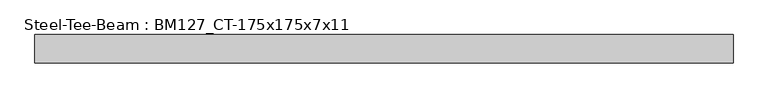
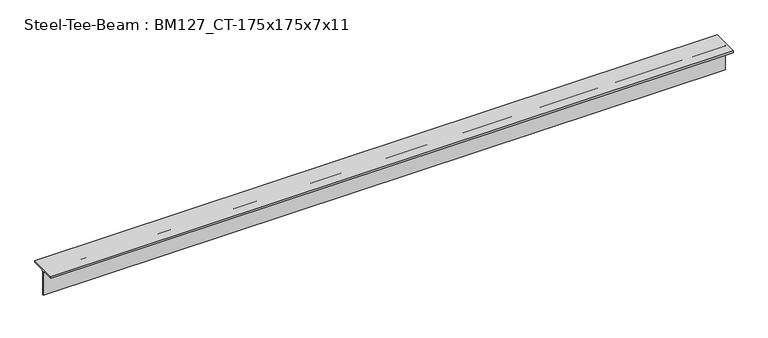
"""IFC4 building model written with IfcOpenShell, lengths in millimetres: beam geometry, Steel-Tee-Beam : BM127_CT-175x175x7x11."""

from ifc_helpers import new_model, si_unit, point, frame, frame_2d, origin, place, context, project, spatial, polyline, circle_curve, trimmed, segment, composite_curve, outline, extrude, source, transform, mapped, element, save


def steel_tee_beam_bm127_ct_175x175x7x11_73a373e1(model_context):
    return source(origin(), model_context, "Body", "SweptSolid", [
        extrude(outline(composite_curve([segment(polyline([(87.5, 87.5), (87.5, 76.5), (17.5, 76.5)]), True, "CONTINUOUS"), segment(trimmed(circle_curve(frame_2d((17.5, 62.5)), 14.0), [point((17.5, 76.5))], [point((3.5, 62.5))], True, "CARTESIAN"), True, "CONTINUOUS"), segment(polyline([(3.5, 62.5), (3.5, -87.5), (-3.5, -87.5), (-3.5, 62.5)]), True, "CONTINUOUS"), segment(trimmed(circle_curve(frame_2d((-17.5, 62.5)), 14.0), [point((-3.5, 62.5))], [point((-17.5, 76.5))], True, "CARTESIAN"), True, "CONTINUOUS"), segment(polyline([(-17.5, 76.5), (-87.5, 76.5), (-87.5, 87.5), (87.5, 87.5)]), True, "CONTINUOUS")], self_intersect=False)), frame((-2105.3835132, 0.0, 0.0), z_axis=(1.0, 0.0, 0.0), x_axis=(0.0, 1.0, 0.0)), (0.0, 0.0, 1.0), 4289.6201558),
    ])


if __name__ == "__main__":
    model = new_model("IFC4")
    model_context = context("Model", 3, world=origin())
    ifc_project = project(units=[si_unit("LENGTHUNIT", "METRE", prefix="MILLI")], contexts=[model_context])
    site = spatial("IfcSite", under=ifc_project)
    building = spatial("IfcBuilding", under=site)
    placement = place(None, origin())
    steel_tee_beam_bm127_ct_175x175x7x11_shape = steel_tee_beam_bm127_ct_175x175x7x11_73a373e1(model_context)
    element("IfcBeam", 1, ObjectType="Steel-Tee-Beam : BM127_CT-175x175x7x11", at=placement, inside=building, context=model_context, shape_type="MappedRepresentation", body=[
        mapped(steel_tee_beam_bm127_ct_175x175x7x11_shape, transform((0.0, 0.0, 0.0), x_axis=(1.0, 0.0, 0.0), y_axis=(0.0, 1.0, 0.0), z_axis=(0.0, 0.0, 1.0))),
    ])
    save(model, "model.ifc")

# Revit data of these elements
# Type "Steel-Tee-Beam : BM127_CT-175x175x7x11"
#   Surface Area = 0.00 m²/m
#   Section Area = 31.57 cm²
#   Mass per Unit Length = 24.80 kg/m
#   Length [instance default] = 1524 mm
#   bf = 175 mm
#   d = 175 mm
#   k = 25 mm
#   kr = 14 mm
#   tf = 11 mm
#   tw = 7 mm
#   hec_material4 [instance default] = none
#   hec_material3 [instance default] = none
#   hec_material2 [instance default] = none
#   hec_material1 [instance default] = none
#   Structural Material [instance default] = Steel, 45-345
#   Assembly Code = ""
# Element 1 (IfcBeam, "Steel-Tee-Beam : BM127_CT-175x175x7x11")
#   hec_material3 = F01AC000-00002_Building/Shelter Fire Proofing Work_Intumescent Coating Type_1 hr. rating (UL 1709))
#   hec_material2 = S01AA010-00002_Main Steel Structure Fabrication Work_Shelter/Building_Steel Painting/Coating_for Fireproofed Steel Surface, Surface Preparation & Primer Coat
#   hec_material1 = S03AA029-00001_Main Steel Structure Erection Work_Shelter/Building_Light Steel
#   Structural Material = S01AA003-00001_Main Steel Structure Fabrication Work_Shelter/Building_Light Steel - Standard
#   Materials on its faces: "S01AA003-00001_Main Steel Structure Fabrication Work_Shelter/Building_Light Steel - Standard"
# Materials
#   "Steel, 45-345": class "Metal", colour RGB 189 187 185, transparency 0, Description = "Steel 345 MPa", Cost = 0
#   "S01AA003-00001_Main Steel Structure Fabrication Work_Shelter/Building_Light Steel - Standard": class "Metal", colour RGB 120 120 120, transparency 0, Comments = "(30KG/M>Weight)", Description = "Structural steel 50ksi", W00) Work Master Code = "S01AA003-00001", W01) Work Master_Lv1 = "Main Steel Structure Fabrication Work", W02) Work Master_Lv2 = "Shelter/Building", W03) Work Master_Spec.1 = "Light Steel - Standard (30KG/M>Weight)", Cost = 0
#   "F01AC000-00002_Building/Shelter Fire Proofing Work_Intumescent Coating Type_1 hr. rating (UL 1709))": class "Metal", colour RGB 255 128 128, transparency 0, Description = "Paint finished steel", W00) Work Master Code = "F01AC000-00002", W01) Work Master_Lv1 = "Building/Shelter Fire Proofing Work", W02) Work Master_Lv2 = "Intumescent Coating Type", W03) Work Master_Spec.1 = "1 hr. rating (UL 1709)", Cost = 0
#   "S01AA010-00002_Main Steel Structure Fabrication Work_Shelter/Building_Steel Painting/Coating_for Fireproofed Steel Surface, Surface Preparation & Primer Coat": class "Metal", colour RGB 120 120 120, transparency 0, Description = "Paint finished steel", W00) Work Master Code = "SS01AA010-00002", W01) Work Master_Lv1 = "Main Steel Structure Fabrication Work", W02) Work Master_Lv2 = "Shelter/Building", W03) Work Master_Spec.1 = "Steel Painting/Coating", W04) Work Master_Spec.2 = "for Fireproofed Steel Surface, Surface Preparation & Primer Coat", Cost = 0
#   "S03AA029-00001_Main Steel Structure Erection Work_Shelter/Building_Light Steel": class "Metal", colour RGB 120 120 120, transparency 0, Comments = "(30KG/M>Weight)", Description = "Structural steel 50ksi", W00) Work Master Code = "S03AA029-00001", W01) Work Master_Lv1 = "Main Steel Structure Erection Work", W02) Work Master_Lv2 = "Shelter/Building", W03) Work Master_Spec.1 = "Light Steel (30KG/M>Weight)", Cost = 0
